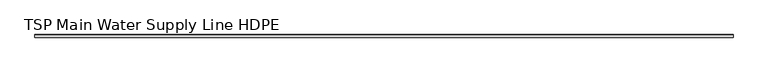
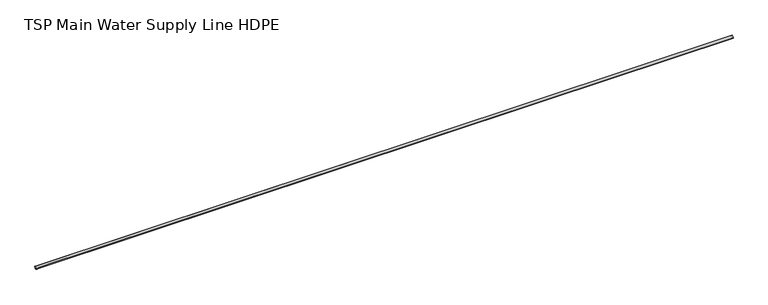
"""IFC4 building model written with IfcOpenShell, lengths in millimetres: flow terminal geometry, TSP Main Water Supply Line HDPE : HDPE Fresh Water Supply."""

from ifc_helpers import new_model, si_unit, point, frame, origin, origin_2d, place, context, project, spatial, circle_curve, trimmed, segment, composite_curve, outline, extrude, source, transform, mapped, element, save


def tsp_main_water_supply_line_hdpe_ff34d8b6(model_context):
    return source(origin(), model_context, "Body", "SweptSolid", [
        extrude(outline(composite_curve([segment(trimmed(circle_curve(origin_2d(), 16.0), [point((-16.0, 0.0))], [point((16.0, 0.0))], False, "CARTESIAN"), True, "CONTINUOUS"), segment(trimmed(circle_curve(origin_2d(), 16.0), [point((16.0, 0.0))], [point((-16.0, 0.0))], False, "CARTESIAN"), True, "CONTINUOUS")], self_intersect=False), holes=[composite_curve([segment(trimmed(circle_curve(origin_2d(), 15.0), [point((-15.0, 0.0))], [point((15.0, 0.0))], True, "CARTESIAN"), True, "CONTINUOUS"), segment(trimmed(circle_curve(origin_2d(), 15.0), [point((15.0, 0.0))], [point((-15.0, 0.0))], True, "CARTESIAN"), True, "CONTINUOUS")], self_intersect=False)]), frame((0.0, 0.0, 0.0), z_axis=(1.0, 0.0, 0.0), x_axis=(0.0, 1.0, 0.0)), (0.0, 0.0, 1.0), 8500.0),
    ])


if __name__ == "__main__":
    model = new_model("IFC4")
    model_context = context("Model", 3, world=origin())
    ifc_project = project(units=[si_unit("LENGTHUNIT", "METRE", prefix="MILLI")], contexts=[model_context])
    site = spatial("IfcSite", under=ifc_project)
    building = spatial("IfcBuilding", under=site)
    placement = place(None, origin())
    tsp_main_water_supply_line_hdpe_shape = tsp_main_water_supply_line_hdpe_ff34d8b6(model_context)
    element("IfcFlowTerminal", 1, ObjectType="TSP Main Water Supply Line HDPE : HDPE Fresh Water Supply", at=placement, inside=building, context=model_context, shape_type="MappedRepresentation", body=[
        mapped(tsp_main_water_supply_line_hdpe_shape, transform((0.0, 0.0, 0.0), x_axis=(1.0, 0.0, 0.0), y_axis=(0.0, 1.0, 0.0), z_axis=(0.0, 0.0, 1.0))),
    ])
    save(model, "model.ifc")

# Revit data of these elements
# Type "TSP Main Water Supply Line HDPE : HDPE Fresh Water Supply"
#   Model = "TSP_110SFWSP"
#   Pipe length [instance default] = 1200 mm
#   Pipe dia = 30 mm
#   built-in parameter 1001306 [instance default] = 3.93701 (stored number, unit not read)
#   Default Elevation = 0
# Element 1 (IfcFlowTerminal, "TSP Main Water Supply Line HDPE : HDPE Fresh Water Supply")
#   Pipe length = 8500 mm
#   built-in parameter 1001306 = 27.8871 (stored number, unit not read)
#   Materials on its faces: "Aluminum, Anodized Blue"
# Materials
#   "Aluminum, Anodized Blue": class "Metal", colour RGB 120 120 120, transparency 0, Description = "Anodized aluminum, blue", Cost = 0
